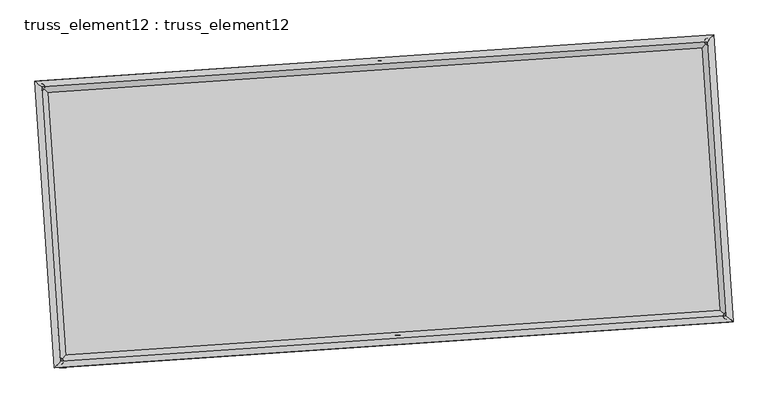
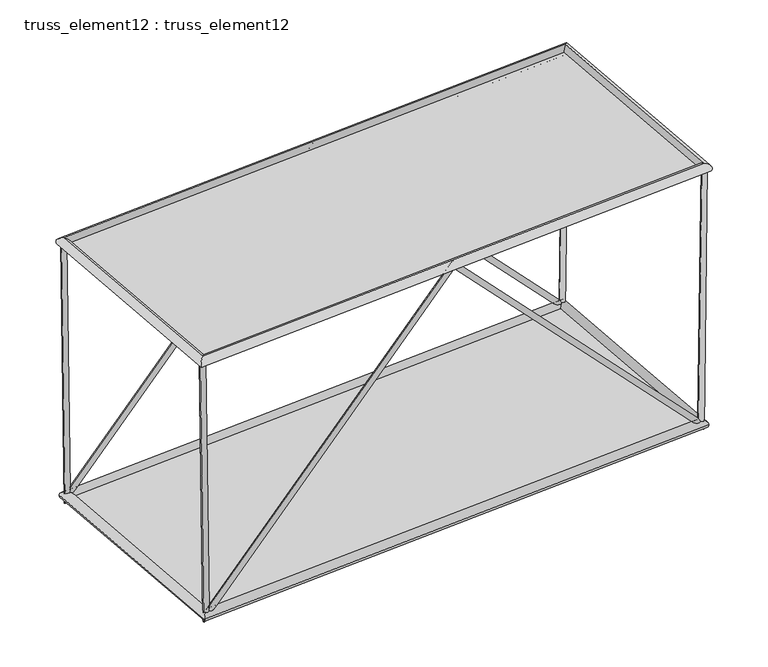
"""IFC4 building model written with IfcOpenShell, lengths in millimetres: plate geometry, truss_element12 : truss_element12."""

import ifcopenshell
import ifcopenshell.guid

model = None  # the IFC model being written
_history = None  # IfcOwnerHistory: only IFC2X3 demands one
_inside = {}  # id of a spatial element -> (the spatial element, [elements in it])
_under = {}  # id of a project, library or spatial element -> (it, [spatial elements below it])
_declared = {}  # id of a project -> (the project, [libraries it declares])
_typed = {}  # id of a type object -> (the type object, [elements of that type])
_made_of = {}  # id of a material, layer set ... -> (it, [elements and type objects made of it])


def new_model(schema):
    """Start an empty IFC model of exactly this schema.

    Asked for "IFC4X3", IfcOpenShell would pick the latest addendum, in which some entities
    have other attributes; the version numbers below select the first issue.
    IFC2X3 requires an IfcOwnerHistory on every rooted entity: one is made here for all.
    """
    global model, _history
    if schema == "IFC4X3":
        model = ifcopenshell.file(schema_version=(4, 3, 0, 0))
    else:
        model = ifcopenshell.file(schema=schema)
    _inside.clear()
    _under.clear()
    _declared.clear()
    _typed.clear()
    _made_of.clear()
    _history = None
    if model.schema == "IFC2X3":
        org = make("IfcOrganization", Name="unknown")
        user = make(
            "IfcPersonAndOrganization",
            ThePerson=make("IfcPerson", FamilyName="unknown"),
            TheOrganization=org,
        )
        app = make(
            "IfcApplication",
            ApplicationDeveloper=org,
            Version="unknown",
            ApplicationFullName="unknown",
            ApplicationIdentifier="unknown",
        )
        _history = make(
            "IfcOwnerHistory",
            OwningUser=user,
            OwningApplication=app,
            ChangeAction="ADDED",
            CreationDate=0,
        )
    return model


def make(cls, **values):
    """One entity of the class cls with the attributes given. An attribute that is None is left unset."""
    return model.create_entity(
        cls, **{name: value for name, value in values.items() if value is not None}
    )


def rooted(cls, **values):
    """An entity with a GlobalId (a new one), such as an element, a storey or a relation."""
    return make(cls, GlobalId=ifcopenshell.guid.new(), OwnerHistory=_history, **values)


def si_unit(unit_type, name, prefix=None):
    """IfcSIUnit, for example si_unit("LENGTHUNIT", "METRE", prefix="MILLI")."""
    return make("IfcSIUnit", UnitType=unit_type, Prefix=prefix, Name=name)


def assignment(units):
    """IfcUnitAssignment: the units of a project."""
    return None if units is None else make("IfcUnitAssignment", Units=units)


def point(xyz):
    """IfcCartesianPoint."""
    return None if xyz is None else make("IfcCartesianPoint", Coordinates=xyz)


def direction(xyz):
    """IfcDirection."""
    return None if xyz is None else make("IfcDirection", DirectionRatios=xyz)


def frame(location, z_axis=None, x_axis=None):
    """IfcAxis2Placement3D, a coordinate frame: its origin and axes. An axis left out is left unset."""
    return make(
        "IfcAxis2Placement3D",
        Location=point(location),
        Axis=direction(z_axis),
        RefDirection=direction(x_axis),
    )


def origin():
    """The frame at (0, 0, 0) with its axes left unset."""
    return frame((0.0, 0.0, 0.0))


def origin_with_axes():
    """The frame at (0, 0, 0) with the z axis (0, 0, 1) and the x axis (1, 0, 0) written out."""
    return frame((0.0, 0.0, 0.0), z_axis=(0.0, 0.0, 1.0), x_axis=(1.0, 0.0, 0.0))


def place(relative_to, where):
    """IfcLocalPlacement: puts the frame where relative to a parent placement (None: the world)."""
    return make(
        "IfcLocalPlacement", PlacementRelTo=relative_to, RelativePlacement=where
    )


def context(
    kind, dimensions, precision=None, world=None, true_north=None, identifier=None
):
    """IfcGeometricRepresentationContext, for example the 3D "Model" context."""
    return make(
        "IfcGeometricRepresentationContext",
        ContextIdentifier=identifier,
        ContextType=kind,
        CoordinateSpaceDimension=dimensions,
        Precision=precision,
        WorldCoordinateSystem=world,
        TrueNorth=true_north,
    )


def project(units=None, contexts=None):
    """IfcProject with its units and contexts."""
    return rooted(
        "IfcProject",
        Name="project",
        RepresentationContexts=contexts,
        UnitsInContext=assignment(units),
    )


def spatial(cls, under=None, at=None, **own):
    """A site, building, storey or space (cls), placed at a placement, below another one or the project."""
    s = rooted(cls, ObjectPlacement=at, **own)
    if under is not None:
        _under.setdefault(under.id(), (under, []))[1].append(s)
    return s


def polyline(points):
    """IfcPolyline through the points."""
    return make("IfcPolyline", Points=[point(p) for p in points])


def circle_curve(where, radius):
    """IfcCircle in the frame where."""
    return make("IfcCircle", Position=where, Radius=radius)


def ellipse_curve(where, semi_axis1, semi_axis2):
    """IfcEllipse in the frame where."""
    return make(
        "IfcEllipse", Position=where, SemiAxis1=semi_axis1, SemiAxis2=semi_axis2
    )


def outline(outer, holes=None, kind="AREA"):
    """IfcArbitraryClosedProfileDef: a profile drawn as a closed curve; with holes, ...WithVoids."""
    if holes is None:
        return make("IfcArbitraryClosedProfileDef", ProfileType=kind, OuterCurve=outer)
    return make(
        "IfcArbitraryProfileDefWithVoids",
        ProfileType=kind,
        OuterCurve=outer,
        InnerCurves=holes,
    )


def extrude(swept, where, along, depth):
    """IfcExtrudedAreaSolid: the profile swept, set in the frame where, extruded along a direction by depth."""
    return make(
        "IfcExtrudedAreaSolid",
        SweptArea=swept,
        Position=where,
        ExtrudedDirection=direction(along),
        Depth=depth,
    )


def shape(context_of_items, identifier, shape_type, items):
    """IfcShapeRepresentation: the items that make up one representation, for example the "Body"."""
    return make(
        "IfcShapeRepresentation",
        ContextOfItems=context_of_items,
        RepresentationIdentifier=identifier,
        RepresentationType=shape_type,
        Items=items,
    )


def source(mapping_origin, context_of_items, identifier, shape_type, items):
    """IfcRepresentationMap: a shape defined once, which mapped items show again and again."""
    return make(
        "IfcRepresentationMap",
        MappingOrigin=mapping_origin,
        MappedRepresentation=shape(context_of_items, identifier, shape_type, items),
    )


def transform(
    local_origin,
    x_axis=None,
    y_axis=None,
    z_axis=None,
    scale=None,
    scale2=None,
    scale3=None,
    uniform=True,
):
    """IfcCartesianTransformationOperator3D, or its non-uniform kind. x_axis, y_axis, z_axis: its Axis1, 2, 3."""
    if uniform:
        return make(
            "IfcCartesianTransformationOperator3D",
            Axis1=direction(x_axis),
            Axis2=direction(y_axis),
            LocalOrigin=point(local_origin),
            Scale=scale,
            Axis3=direction(z_axis),
        )
    return make(
        "IfcCartesianTransformationOperator3DnonUniform",
        Axis1=direction(x_axis),
        Axis2=direction(y_axis),
        LocalOrigin=point(local_origin),
        Scale=scale,
        Axis3=direction(z_axis),
        Scale2=scale2,
        Scale3=scale3,
    )


def mapped(mapping_source, mapping_target):
    """IfcMappedItem: shows the shape of a source again, moved by a transform."""
    return make(
        "IfcMappedItem", MappingSource=mapping_source, MappingTarget=mapping_target
    )


def made_of(thing, what):
    """Note that an element or type object is made of a material, layer set ...; save() writes the relation."""
    if what is not None:
        _made_of.setdefault(what.id(), (what, []))[1].append(thing)
    return thing


def element(
    cls,
    number,
    at=None,
    inside=None,
    cuts=None,
    type_object=None,
    material=None,
    context=None,
    identifier="Body",
    shape_type=None,
    held_by="IfcProductDefinitionShape",
    body=None,
    shapes=None,
    **own,
):
    """One element of the class cls, such as IfcWall. Its Tag is "e" and its number.

    at: its placement. inside: the storey or other place that contains it. cuts: it is an
    opening in that element (IfcRelVoidsElement). A single representation is given by context,
    identifier, shape_type and body (its items); several are given by shapes. held_by: the class
    of the entity that holds the representations. save() writes the other relations.
    """
    e = rooted(cls, Tag="e%d" % number, ObjectPlacement=at, **own)
    if body is not None:
        shapes = [shape(context, identifier, shape_type, body)]
    if shapes is not None:
        e.Representation = make(held_by, Representations=shapes)
    if inside is not None:
        _inside.setdefault(inside.id(), (inside, []))[1].append(e)
    if cuts is not None:
        rooted(
            "IfcRelVoidsElement", RelatingBuildingElement=cuts, RelatedOpeningElement=e
        )
    if type_object is not None:
        _typed.setdefault(type_object.id(), (type_object, []))[1].append(e)
    return made_of(e, material)


def aggregate(whole, parts):
    """IfcRelAggregates: a whole, such as a stair, and the parts it consists of."""
    return rooted("IfcRelAggregates", RelatingObject=whole, RelatedObjects=parts)


def save(model, path):
    """Write the relations noted so far, then the file.

    IfcRelAggregates (storeys below a building ...), IfcRelContainedInSpatialStructure (elements
    in a storey), IfcRelDefinesByType, IfcRelAssociatesMaterial and IfcRelDeclares: one each for
    every whole, place, type object, material and project.
    """
    for whole, parts in _under.values():
        aggregate(whole, parts)
    for where, things in _inside.values():
        rooted(
            "IfcRelContainedInSpatialStructure",
            RelatedElements=things,
            RelatingStructure=where,
        )
    for kind, things in _typed.values():
        rooted("IfcRelDefinesByType", RelatedObjects=things, RelatingType=kind)
    for what, things in _made_of.values():
        rooted("IfcRelAssociatesMaterial", RelatedObjects=things, RelatingMaterial=what)
    for by, libraries in _declared.values():
        rooted("IfcRelDeclares", RelatingContext=by, RelatedDefinitions=libraries)
    model.write(path)


def plane_surface(at):
    """IfcPlane: the flat surface through the origin of the frame at, square to its z axis."""
    return make("IfcPlane", Position=at)


def cylinder_surface(at, radius):
    """IfcCylindricalSurface: all points at the distance radius from the z axis of the frame at."""
    return make("IfcCylindricalSurface", Position=at, Radius=radius)


def advanced_brep(points, edges, surfaces, faces):
    """IfcAdvancedBrep: a solid bounded by faces that lie on surfaces and meet in shared edges.

    An edge is (start, end): straight between two places in points (the first is 0);
    or (start, end, curve); or (start, end, curve, False) where it runs against its curve.
    A face is (place in surfaces, loops), or (place, loops, False) where it looks against
    its surface's normal. A loop lists edges by number (the first is 1), with a minus sign
    where the edge is run from its end to its start. The first loop is the outer one.
    """
    corners = [point(p) for p in points]
    vertices = [make("IfcVertexPoint", VertexGeometry=c) for c in corners]
    made = []
    for start, end, *more in edges:
        made.append(
            make(
                "IfcEdgeCurve",
                EdgeStart=vertices[start],
                EdgeEnd=vertices[end],
                EdgeGeometry=more[0] if more else make("IfcPolyline", Points=[corners[start], corners[end]]),
                SameSense=more[1] if len(more) > 1 else True,
            )
        )
    hull = []
    for where, loops, *sense in faces:
        bounds = []
        for j, loop in enumerate(loops):
            ring = [make("IfcOrientedEdge", EdgeElement=made[abs(k) - 1], Orientation=k > 0) for k in loop]
            bounds.append(
                make(
                    "IfcFaceOuterBound" if j == 0 else "IfcFaceBound",
                    Bound=make("IfcEdgeLoop", EdgeList=ring),
                    Orientation=True,
                )
            )
        hull.append(make("IfcAdvancedFace", Bounds=bounds, FaceSurface=surfaces[where], SameSense=sense[0] if sense else True))
    return make("IfcAdvancedBrep", Outer=make("IfcClosedShell", CfsFaces=hull))


def truss_element12_truss_element12_8e82c5bd(model_context):
    return source(origin(), model_context, "Body", "SolidModel", [
        advanced_brep(
        [(-3731.8869442, 2271.6592401, 5000.2192941), (-3830.9813422, 2258.2985761, 4998.880287), (-3666.5774651, 2276.1124452, 122.499402), (-3762.4094178, 2262.9742349, -122.499402), (1063.116068, 2598.6122679, 5071.6784027), (1063.5732809, 2592.0396499, 4927.4371453), (5793.9872263, 2921.1923885, 122.5077755), (5890.7737507, 2921.1881, -122.5077755), (5858.1279304, 2925.5658993, 5000.2232822), (5958.1190537, 2925.7801202, 4998.9082326)],
        [
            (0, 1, circle_curve(frame((-3781.4341432, 2264.9789081, 4999.5497906), z_axis=(-0.013388140355827645, -0.0009128863977796117, 0.9999099581143482), x_axis=(-0.13360683337915732, 0.9910340218161442, -0.0008841251678223183)), 50.0)),
            (1, 0, circle_curve(frame((-3781.4341432, 2264.9789081, 4999.5497906), z_axis=(-0.013388140355827645, -0.0009128863977796117, 0.9999099581143482), x_axis=(-0.13360683337915732, 0.9910340218161442, -0.0008841251678223183)), 50.0)),
            (0, 2),
            (2, 3, ellipse_curve(frame((-3714.4934414, 2269.54334, 0.0), z_axis=(-0.9282671693555781, -0.06329500960449433, 0.36648847738469154), x_axis=(0.36563946873946984, 0.02493156544759802, 0.9304225899795482)), 131.9466513, 50.0)),
            (3, 1),
            (3, 2, ellipse_curve(frame((-3714.4934414, 2269.54334, 0.0), z_axis=(-0.9282671693555781, -0.06329500960449433, 0.36648847738469154), x_axis=(0.36563946873946984, 0.02493156544759802, 0.9304225899795482)), 131.9466513, 50.0)),
            (2, 4),
            (4, 5, ellipse_curve(frame((1063.3446744, 2595.3259589, 4999.557774), z_axis=(-0.9976833941197891, -0.0680282380953912, -6.260394869337924e-05), x_axis=(6.245892014005556e-05, 4.258836337772687e-06, -0.9999999980403728)), 72.2776719, 50.0)),
            (5, 3),
            (5, 4, ellipse_curve(frame((1063.3446744, 2595.3259589, 4999.557774), z_axis=(-0.9976833941197891, -0.0680282380953912, -6.260394869337924e-05), x_axis=(6.245892014005556e-05, 4.258836337772687e-06, -0.9999999980403728)), 72.2776719, 50.0)),
            (4, 6),
            (6, 7, ellipse_curve(frame((5842.3804885, 2921.1902443, 0.0), z_axis=(-0.9282003652529641, -0.06329045448668236, -0.36665842457951714), x_axis=(-0.36580902223395634, -0.024943126655857368, 0.9303556307589407)), 131.9651677, 50.0)),
            (7, 5),
            (7, 6, ellipse_curve(frame((5842.3804885, 2921.1902443, 0.0), z_axis=(-0.9282003652529641, -0.06329045448668236, -0.36665842457951714), x_axis=(-0.36580902223395634, -0.024943126655857368, 0.9303556307589407)), 131.9651677, 50.0)),
            (8, 9, circle_curve(frame((5908.1234921, 2925.6730098, 4999.5657574), z_axis=(0.013148600710357648, 0.0008965530999268896, 0.9999131514746162), x_axis=(-0.002153813196862378, 0.9999973035626637, -0.0008683064638333599)), 50.0)),
            (9, 8, circle_curve(frame((5908.1234921, 2925.6730098, 4999.5657574), z_axis=(0.013148600710357648, 0.0008965530999268896, 0.9999131514746162), x_axis=(-0.002153813196862378, 0.9999973035626637, -0.0008683064638333599)), 50.0)),
            (6, 8),
            (9, 7),
        ],
        [
            plane_surface(frame((-3781.4341432, 2314.9788872, 4999.595439), z_axis=(-0.01338814035582826, -0.0009128863977758225, 0.9999099581143482), x_axis=(0.9999103748325711, -1.2222946706330628e-05, 0.013388134776246131))),
            cylinder_surface(frame((-3781.4341432, 2264.9789081, 4999.5497906), z_axis=(-0.013388140355827645, -0.0009128863977796117, 0.9999099581143482), x_axis=(-0.13360683337915732, 0.9910340218161442, -0.0008841251678223183)), 50.0),
            cylinder_surface(frame((-3714.4934414, 2269.54334, 0.0), z_axis=(-0.6901288948828247, -0.04705726591652543, -0.722154915632562), x_axis=(-0.02041150749335854, 0.9987523807925791, -0.04557468840270432)), 50.0),
            cylinder_surface(frame((1063.3446744, 2595.3259589, 4999.557774), z_axis=(-0.6902190995054749, -0.04706341662684697, 0.7220682997426625), x_axis=(-0.11534365552593137, 0.9922793184891172, -0.04558064532988163)), 50.0),
            plane_surface(frame((5908.1234921, 2875.6730298, 4999.6105889), z_axis=(0.01314860071035912, 0.0008965530999253627, 0.9999131514746162), x_axis=(0.9999135534131737, -1.1789437882825396e-05, -0.013148595424972613))),
            cylinder_surface(frame((5842.3804885, 2921.1902443, 0.0), z_axis=(-0.013148600710357651, -0.0008965530999268898, -0.9999131514746165), x_axis=(-0.002153813196862378, 0.9999973035626637, -0.0008683064638333599)), 50.0),
        ],
        [
            (0, [[1, 2]]),
            (1, [[-1, 3, 4, 5]]),
            (1, [[-2, -5, 6, -3]]),
            (2, [[-4, 7, 8, 9]]),
            (2, [[-6, -9, 10, -7]]),
            (3, [[-8, 11, 12, 13]]),
            (3, [[-10, -13, 14, -11]]),
            (4, [[15, 16]]),
            (5, [[-12, 17, -16, 18]]),
            (5, [[-14, -18, -15, -17]]),
        ],
    ),
        advanced_brep(
        [(-3459.7739913, -1719.0743442, 5000.2192941), (-3558.8683893, -1732.4350082, 4998.880287), (-3394.4645122, -1714.6211391, 122.499402), (-3490.2964649, -1727.7593494, -122.499402), (1335.2290209, -1392.1213164, 5071.6784027), (1335.6862338, -1398.6939344, 4927.4371453), (6066.1001792, -1069.5411958, 122.5077755), (6162.8867037, -1069.5454843, -122.5077755), (6130.2408833, -1065.167685, 5000.2232822), (6230.2320067, -1064.9534641, 4998.9082326)],
        [
            (0, 1, circle_curve(frame((-3509.3211903, -1725.7546762, 4999.5497906), z_axis=(-0.013388140355828339, -0.0009128863977796623, 0.9999099581143481), x_axis=(-0.13360683337915777, 0.9910340218161441, -0.0008841251678223668)), 50.0)),
            (1, 0, circle_curve(frame((-3509.3211903, -1725.7546762, 4999.5497906), z_axis=(-0.013388140355828339, -0.0009128863977796623, 0.9999099581143481), x_axis=(-0.13360683337915777, 0.9910340218161441, -0.0008841251678223668)), 50.0)),
            (0, 2),
            (2, 3, ellipse_curve(frame((-3442.3804885, -1721.1902443, 0.0), z_axis=(-0.9282671693555784, -0.06329500960449469, 0.3664884773846907), x_axis=(0.36563946873946884, 0.024931565447598097, 0.9304225899795485)), 131.9466513, 50.0)),
            (3, 1),
            (3, 2, ellipse_curve(frame((-3442.3804885, -1721.1902443, 0.0), z_axis=(-0.9282671693555784, -0.06329500960449469, 0.3664884773846907), x_axis=(0.36563946873946884, 0.024931565447598097, 0.9304225899795485)), 131.9466513, 50.0)),
            (2, 4),
            (4, 5, ellipse_curve(frame((1335.4576273, -1395.4076254, 4999.557774), z_axis=(-0.9976833941197891, -0.06802823809539131, -6.260394869402122e-05), x_axis=(6.245892014067052e-05, 4.258836337570893e-06, -0.9999999980403728)), 72.2776719, 50.0)),
            (5, 3),
            (5, 4, ellipse_curve(frame((1335.4576273, -1395.4076254, 4999.557774), z_axis=(-0.9976833941197891, -0.06802823809539131, -6.260394869402122e-05), x_axis=(6.245892014067052e-05, 4.258836337570893e-06, -0.9999999980403728)), 72.2776719, 50.0)),
            (4, 6),
            (6, 7, ellipse_curve(frame((6114.4934414, -1069.54334, 0.0), z_axis=(-0.9282003652529639, -0.06329045448668222, -0.3666584245795172), x_axis=(-0.36580902223395667, -0.02494312665585735, 0.9303556307589408)), 131.9651677, 50.0)),
            (7, 5),
            (7, 6, ellipse_curve(frame((6114.4934414, -1069.54334, 0.0), z_axis=(-0.9282003652529639, -0.06329045448668222, -0.3666584245795172), x_axis=(-0.36580902223395667, -0.02494312665585735, 0.9303556307589408)), 131.9651677, 50.0)),
            (8, 9, circle_curve(frame((6180.236445, -1065.0605745, 4999.5657574), z_axis=(0.013148600710357764, 0.0008965530999268809, 0.9999131514746162), x_axis=(-0.002153813196862232, 0.9999973035626636, -0.0008683064638333527)), 50.0)),
            (9, 8, circle_curve(frame((6180.236445, -1065.0605745, 4999.5657574), z_axis=(0.013148600710357764, 0.0008965530999268809, 0.9999131514746162), x_axis=(-0.002153813196862232, 0.9999973035626636, -0.0008683064638333527)), 50.0)),
            (6, 8),
            (9, 7),
        ],
        [
            plane_surface(frame((-3509.3211903, -1675.7546971, 4999.595439), z_axis=(-0.01338814035582826, -0.0009128863977758175, 0.9999099581143482), x_axis=(0.9999103748325711, -1.2222946706330628e-05, 0.013388134776246131))),
            cylinder_surface(frame((-3509.3211903, -1725.7546762, 4999.5497906), z_axis=(-0.013388140355828339, -0.0009128863977796623, 0.9999099581143481), x_axis=(-0.13360683337915777, 0.9910340218161441, -0.0008841251678223668)), 50.0),
            cylinder_surface(frame((-3442.3804885, -1721.1902443, 0.0), z_axis=(-0.6901288948828239, -0.04705726591652563, -0.7221549156325626), x_axis=(-0.02041150749335876, 0.9987523807925791, -0.04557468840270436)), 50.0),
            cylinder_surface(frame((1335.4576273, -1395.4076254, 4999.557774), z_axis=(-0.690219099505475, -0.047063416626846884, 0.7220682997426622), x_axis=(-0.11534365552593126, 0.9922793184891172, -0.045580645329881674)), 50.0),
            plane_surface(frame((6180.236445, -1115.0605545, 4999.6105889), z_axis=(0.01314860071035912, 0.0008965530999253614, 0.9999131514746162), x_axis=(0.9999135534131737, -1.1789437883269485e-05, -0.013148595424972613))),
            cylinder_surface(frame((6114.4934414, -1069.54334, 0.0), z_axis=(-0.013148600710357764, -0.0008965530999268809, -0.9999131514746162), x_axis=(-0.002153813196862232, 0.9999973035626636, -0.0008683064638333527)), 50.0),
        ],
        [
            (0, [[1, 2]]),
            (1, [[-1, 3, 4, 5]]),
            (1, [[-2, -5, 6, -3]]),
            (2, [[-4, 7, 8, 9]]),
            (2, [[-6, -9, 10, -7]]),
            (3, [[-8, 11, 12, 13]]),
            (3, [[-10, -13, 14, -11]]),
            (4, [[15, 16]]),
            (5, [[-12, 17, -16, 18]]),
            (5, [[-14, -18, -15, -17]]),
        ],
    ),
        advanced_brep(
        [(-3509.3170033, -1725.7500357, 4909.5497907), (-3509.3253772, -1725.7593168, 5089.5497905), (-3781.4389213, 2264.9829373, 5089.5497905), (-3781.4293651, 2264.9748788, 4909.5497907), (5908.1273838, 2925.6776302, 5089.5657573), (5908.1196003, 2925.6683893, 4909.5657575), (6180.2409278, -1065.0646239, 5089.5657573), (6180.2319621, -1065.0565252, 4909.5657575)],
        [
            (0, 1, ellipse_curve(frame((-3509.3211903, -1725.7546762, 4999.5497906), z_axis=(-0.7535719234045052, 0.6573654662781452, -1.1624966718516507e-06), x_axis=(-0.6573654662771268, -0.7535719234053935, -1.1624966718515976e-06)), 127.2792206, 90.0)),
            (1, 2),
            (2, 3, ellipse_curve(frame((-3781.4341432, 2264.9789081, 4999.5497906), z_axis=(-0.6573654662771266, -0.7535719234053936, -1.1624966705901006e-06), x_axis=(0.7535719234045052, -0.6573654662781453, 1.1624966705901538e-06)), 127.2792206, 90.0)),
            (3, 0),
            (1, 0, ellipse_curve(frame((-3509.3211903, -1725.7546762, 4999.5497906), z_axis=(-0.7535719234045052, 0.6573654662781452, -1.1624966718516507e-06), x_axis=(-0.6573654662771268, -0.7535719234053935, -1.1624966718515976e-06)), 127.2792206, 90.0)),
            (3, 2, ellipse_curve(frame((-3781.4341432, 2264.9789081, 4999.5497906), z_axis=(-0.6573654662771266, -0.7535719234053936, -1.1624966705901006e-06), x_axis=(0.7535719234045052, -0.6573654662781453, 1.1624966705901538e-06)), 127.2792206, 90.0)),
            (2, 4),
            (4, 5, ellipse_curve(frame((5908.1234921, 2925.6730098, 4999.5657574), z_axis=(-0.7535719234045045, 0.657365466278146, -1.1624966736529165e-06), x_axis=(-0.6573654662771276, -0.7535719234053929, -1.1624966675273385e-06)), 127.2792206, 90.0)),
            (5, 3),
            (5, 4, ellipse_curve(frame((5908.1234921, 2925.6730098, 4999.5657574), z_axis=(-0.7535719234045045, 0.657365466278146, -1.1624966736529165e-06), x_axis=(-0.6573654662771276, -0.7535719234053929, -1.1624966675273385e-06)), 127.2792206, 90.0)),
            (4, 6),
            (6, 7, ellipse_curve(frame((6180.236445, -1065.0605745, 4999.5657574), z_axis=(0.6573654662771274, 0.7535719234053929, 1.1624966687888353e-06), x_axis=(-0.7535719234045046, 0.657365466278146, -1.1624966749144135e-06)), 127.2792206, 90.0)),
            (7, 5),
            (7, 6, ellipse_curve(frame((6180.236445, -1065.0605745, 4999.5657574), z_axis=(0.6573654662771274, 0.7535719234053929, 1.1624966687888353e-06), x_axis=(-0.7535719234045046, 0.657365466278146, -1.1624966749144135e-06)), 127.2792206, 90.0)),
            (6, 1),
            (0, 7),
        ],
        [
            cylinder_surface(frame((-3509.3211903, -1725.7546762, 4999.5497906), z_axis=(0.06802823822870178, -0.9976833960748765, 0.0), x_axis=(-0.9976833948316877, -0.06802823814393347, -4.992144956552851e-05)), 90.0),
            cylinder_surface(frame((-3781.4341432, 2264.9789081, 4999.5497906), z_axis=(-0.9976833960735284, -0.06802823822861073, -1.644018557762127e-06), x_axis=(-0.06802823807024047, 0.9976833949176204, -4.8277431009682214e-05)), 90.0),
            cylinder_surface(frame((5908.1234921, 2925.6730098, 4999.5657574), z_axis=(-0.06802823822869981, 0.9976833960748768, 0.0), x_axis=(0.9976833949900581, 0.06802823815473016, -4.663341244950445e-05)), 90.0),
            cylinder_surface(frame((6180.236445, -1065.0605745, 4999.5657574), z_axis=(0.9976833960735283, 0.06802823822861062, 1.6440185595461528e-06), x_axis=(0.06802823822861061, -0.9976833949068217, -4.827743100280322e-05)), 90.0),
        ],
        [
            (0, [[1, 2, 3, 4]]),
            (0, [[5, -4, 6, -2]]),
            (1, [[-3, 7, 8, 9]]),
            (1, [[-6, -9, 10, -7]]),
            (2, [[-8, 11, 12, 13]]),
            (2, [[-10, -13, 14, -11]]),
            (3, [[-12, 15, -1, 16]]),
            (3, [[-14, -16, -5, -15]]),
        ],
    ),
        advanced_brep(
        [(-3358.7115243, -1625.2761972, 0.0), (-3526.0494527, -1817.1042913, 0.0), (-3810.4074885, 2353.2123043, 0.0), (-3618.5793943, 2185.8743758, 0.0), (5926.0494527, 3017.1042913, 0.0), (5758.7115243, 2825.2761972, 0.0), (6210.4074885, -1153.2123043, 0.0), (6018.5793943, -985.8743758, 0.0)],
        [
            (0, 1, ellipse_curve(frame((-3442.3804885, -1721.1902443, 0.0), z_axis=(-0.7535719234054579, 0.6573654662780808, 0.0), x_axis=(-0.6573654662780808, -0.753571923405458, 0.0)), 127.2792206, 90.0)),
            (1, 2),
            (2, 3, ellipse_curve(frame((-3714.4934414, 2269.54334, 0.0), z_axis=(-0.6573654662780806, -0.7535719234054582, 0.0), x_axis=(0.7535719234054582, -0.6573654662780805, 0.0)), 127.2792206, 90.0)),
            (3, 0),
            (1, 0, ellipse_curve(frame((-3442.3804885, -1721.1902443, 0.0), z_axis=(-0.7535719234054579, 0.6573654662780808, 0.0), x_axis=(-0.6573654662780808, -0.753571923405458, 0.0)), 127.2792206, 90.0)),
            (3, 2, ellipse_curve(frame((-3714.4934414, 2269.54334, 0.0), z_axis=(-0.6573654662780806, -0.7535719234054582, 0.0), x_axis=(0.7535719234054582, -0.6573654662780805, 0.0)), 127.2792206, 90.0)),
            (2, 4),
            (4, 5, ellipse_curve(frame((5842.3804885, 2921.1902443, 0.0), z_axis=(-0.7535719234054572, 0.6573654662780816, 0.0), x_axis=(-0.6573654662780819, -0.7535719234054571, 0.0)), 127.2792206, 90.0)),
            (5, 3),
            (5, 4, ellipse_curve(frame((5842.3804885, 2921.1902443, 0.0), z_axis=(-0.7535719234054572, 0.6573654662780816, 0.0), x_axis=(-0.6573654662780819, -0.7535719234054571, 0.0)), 127.2792206, 90.0)),
            (4, 6),
            (6, 7, ellipse_curve(frame((6114.4934414, -1069.54334, 0.0), z_axis=(0.6573654662780819, 0.7535719234054572, 0.0), x_axis=(-0.7535719234054573, 0.6573654662780816, 0.0)), 127.2792206, 90.0)),
            (7, 5),
            (7, 6, ellipse_curve(frame((6114.4934414, -1069.54334, 0.0), z_axis=(0.6573654662780819, 0.7535719234054572, 0.0), x_axis=(-0.7535719234054573, 0.6573654662780816, 0.0)), 127.2792206, 90.0)),
            (6, 1),
            (0, 7),
        ],
        [
            cylinder_surface(frame((-3442.3804885, -1721.1902443, 0.0), z_axis=(0.06802823822870138, -0.9976833960748765, 0.0), x_axis=(-0.9976833960748765, -0.06802823822870138, 0.0)), 90.0),
            cylinder_surface(frame((-3714.4934414, 2269.54334, 0.0), z_axis=(-0.9976833960748767, -0.0680282382287016, 0.0), x_axis=(-0.0680282382287016, 0.9976833960748767, 0.0)), 90.0),
            cylinder_surface(frame((5842.3804885, 2921.1902443, 0.0), z_axis=(-0.06802823822869875, 0.9976833960748769, 0.0), x_axis=(0.9976833960748769, 0.06802823822869875, 0.0)), 90.0),
            cylinder_surface(frame((6114.4934414, -1069.54334, 0.0), z_axis=(0.9976833960748767, 0.06802823822870119, 0.0), x_axis=(0.06802823822870119, -0.9976833960748767, 0.0)), 90.0),
        ],
        [
            (0, [[1, 2, 3, 4]]),
            (0, [[5, -4, 6, -2]]),
            (1, [[-3, 7, 8, 9]]),
            (1, [[-6, -9, 10, -7]]),
            (2, [[-8, 11, 12, 13]]),
            (2, [[-10, -13, 14, -11]]),
            (3, [[-12, 15, -1, 16]]),
            (3, [[-14, -16, -5, -15]]),
        ],
    ),
        extrude(outline(polyline([(-3442.3804885, -1721.1902443), (-3714.4934414, 2269.54334), (5842.3804885, 2921.1902443), (6114.4934414, -1069.54334), (-3442.3804885, -1721.1902443)])), origin_with_axes(), (0.0, 0.0, 1.0), 20.0),
        extrude(outline(polyline([(-2000.0, 4856.0283119), (2000.0, 4856.0283119), (2000.0, -4856.0283119), (-2000.0, -4856.0283119), (-2000.0, 4856.0283119)])), frame((1199.4011509, 599.9591668, 4999.557774), z_axis=(-1.6402100179182737e-06, -1.1183968609984865e-07, 0.9999999999986486), x_axis=(-0.06802823822870034, 0.9976833960748767, 0.0)), (0.0, 0.0, 1.0), 20.0),
    ])


if __name__ == "__main__":
    model = new_model("IFC4")
    model_context = context("Model", 3, world=origin())
    ifc_project = project(units=[si_unit("LENGTHUNIT", "METRE", prefix="MILLI")], contexts=[model_context])
    site = spatial("IfcSite", under=ifc_project)
    building = spatial("IfcBuilding", under=site)
    placement = place(None, origin())
    truss_element12_truss_element12_shape = truss_element12_truss_element12_8e82c5bd(model_context)
    element("IfcPlate", 1, ObjectType="truss_element12 : truss_element12", at=placement, inside=building, context=model_context, shape_type="MappedRepresentation", body=[
        mapped(truss_element12_truss_element12_shape, transform((0.0, 0.0, 0.0), x_axis=(1.0, 0.0, 0.0), y_axis=(0.0, 1.0, 0.0), z_axis=(0.0, 0.0, 1.0))),
    ])
    save(model, "model.ifc")

# Revit data of these elements
# Type "truss_element12 : truss_element12"
#   steellbar1 = 90 mm
#   steelbar2 = 50 mm
#   offset1 = 5000 mm
#   M = Default Roof
# Element 1 (IfcPlate, "truss_element12 : truss_element12")
#   Materials on its faces: "Default Roof"
# Materials
#   "Default Roof": class "Miscellaneous", colour RGB 0 127 0, transparency 0, Comments = "Rendering appearance not upgraded Rendering appearance not upgraded ", Cost = 0
